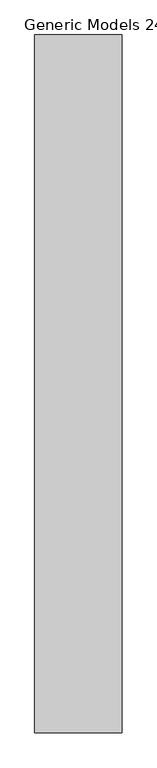
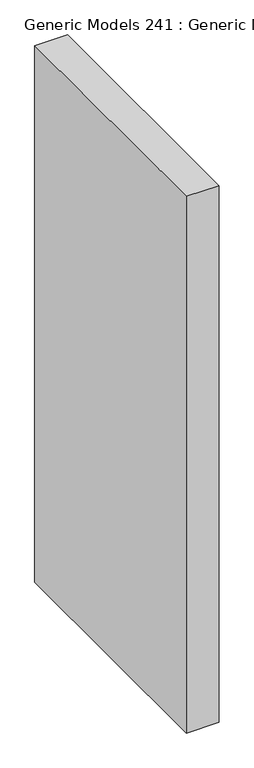
"""IFC4 building model written with IfcOpenShell, lengths in millimetres: proxy geometry, Generic Models 241 : Generic Models 1."""

import ifcopenshell
import ifcopenshell.guid

model = None  # the IFC model being written
_history = None  # IfcOwnerHistory: only IFC2X3 demands one
_inside = {}  # id of a spatial element -> (the spatial element, [elements in it])
_under = {}  # id of a project, library or spatial element -> (it, [spatial elements below it])
_declared = {}  # id of a project -> (the project, [libraries it declares])
_typed = {}  # id of a type object -> (the type object, [elements of that type])
_made_of = {}  # id of a material, layer set ... -> (it, [elements and type objects made of it])


def new_model(schema):
    """Start an empty IFC model of exactly this schema.

    Asked for "IFC4X3", IfcOpenShell would pick the latest addendum, in which some entities
    have other attributes; the version numbers below select the first issue.
    IFC2X3 requires an IfcOwnerHistory on every rooted entity: one is made here for all.
    """
    global model, _history
    if schema == "IFC4X3":
        model = ifcopenshell.file(schema_version=(4, 3, 0, 0))
    else:
        model = ifcopenshell.file(schema=schema)
    _inside.clear()
    _under.clear()
    _declared.clear()
    _typed.clear()
    _made_of.clear()
    _history = None
    if model.schema == "IFC2X3":
        org = make("IfcOrganization", Name="unknown")
        user = make(
            "IfcPersonAndOrganization",
            ThePerson=make("IfcPerson", FamilyName="unknown"),
            TheOrganization=org,
        )
        app = make(
            "IfcApplication",
            ApplicationDeveloper=org,
            Version="unknown",
            ApplicationFullName="unknown",
            ApplicationIdentifier="unknown",
        )
        _history = make(
            "IfcOwnerHistory",
            OwningUser=user,
            OwningApplication=app,
            ChangeAction="ADDED",
            CreationDate=0,
        )
    return model


def make(cls, **values):
    """One entity of the class cls with the attributes given. An attribute that is None is left unset."""
    return model.create_entity(
        cls, **{name: value for name, value in values.items() if value is not None}
    )


def rooted(cls, **values):
    """An entity with a GlobalId (a new one), such as an element, a storey or a relation."""
    return make(cls, GlobalId=ifcopenshell.guid.new(), OwnerHistory=_history, **values)


def si_unit(unit_type, name, prefix=None):
    """IfcSIUnit, for example si_unit("LENGTHUNIT", "METRE", prefix="MILLI")."""
    return make("IfcSIUnit", UnitType=unit_type, Prefix=prefix, Name=name)


def assignment(units):
    """IfcUnitAssignment: the units of a project."""
    return None if units is None else make("IfcUnitAssignment", Units=units)


def point(xyz):
    """IfcCartesianPoint."""
    return None if xyz is None else make("IfcCartesianPoint", Coordinates=xyz)


def direction(xyz):
    """IfcDirection."""
    return None if xyz is None else make("IfcDirection", DirectionRatios=xyz)


def frame(location, z_axis=None, x_axis=None):
    """IfcAxis2Placement3D, a coordinate frame: its origin and axes. An axis left out is left unset."""
    return make(
        "IfcAxis2Placement3D",
        Location=point(location),
        Axis=direction(z_axis),
        RefDirection=direction(x_axis),
    )


def origin():
    """The frame at (0, 0, 0) with its axes left unset."""
    return frame((0.0, 0.0, 0.0))


def place(relative_to, where):
    """IfcLocalPlacement: puts the frame where relative to a parent placement (None: the world)."""
    return make(
        "IfcLocalPlacement", PlacementRelTo=relative_to, RelativePlacement=where
    )


def context(
    kind, dimensions, precision=None, world=None, true_north=None, identifier=None
):
    """IfcGeometricRepresentationContext, for example the 3D "Model" context."""
    return make(
        "IfcGeometricRepresentationContext",
        ContextIdentifier=identifier,
        ContextType=kind,
        CoordinateSpaceDimension=dimensions,
        Precision=precision,
        WorldCoordinateSystem=world,
        TrueNorth=true_north,
    )


def project(units=None, contexts=None):
    """IfcProject with its units and contexts."""
    return rooted(
        "IfcProject",
        Name="project",
        RepresentationContexts=contexts,
        UnitsInContext=assignment(units),
    )


def spatial(cls, under=None, at=None, **own):
    """A site, building, storey or space (cls), placed at a placement, below another one or the project."""
    s = rooted(cls, ObjectPlacement=at, **own)
    if under is not None:
        _under.setdefault(under.id(), (under, []))[1].append(s)
    return s


def polyline(points):
    """IfcPolyline through the points."""
    return make("IfcPolyline", Points=[point(p) for p in points])


def outline(outer, holes=None, kind="AREA"):
    """IfcArbitraryClosedProfileDef: a profile drawn as a closed curve; with holes, ...WithVoids."""
    if holes is None:
        return make("IfcArbitraryClosedProfileDef", ProfileType=kind, OuterCurve=outer)
    return make(
        "IfcArbitraryProfileDefWithVoids",
        ProfileType=kind,
        OuterCurve=outer,
        InnerCurves=holes,
    )


def extrude(swept, where, along, depth):
    """IfcExtrudedAreaSolid: the profile swept, set in the frame where, extruded along a direction by depth."""
    return make(
        "IfcExtrudedAreaSolid",
        SweptArea=swept,
        Position=where,
        ExtrudedDirection=direction(along),
        Depth=depth,
    )


def shape(context_of_items, identifier, shape_type, items):
    """IfcShapeRepresentation: the items that make up one representation, for example the "Body"."""
    return make(
        "IfcShapeRepresentation",
        ContextOfItems=context_of_items,
        RepresentationIdentifier=identifier,
        RepresentationType=shape_type,
        Items=items,
    )


def source(mapping_origin, context_of_items, identifier, shape_type, items):
    """IfcRepresentationMap: a shape defined once, which mapped items show again and again."""
    return make(
        "IfcRepresentationMap",
        MappingOrigin=mapping_origin,
        MappedRepresentation=shape(context_of_items, identifier, shape_type, items),
    )


def transform(
    local_origin,
    x_axis=None,
    y_axis=None,
    z_axis=None,
    scale=None,
    scale2=None,
    scale3=None,
    uniform=True,
):
    """IfcCartesianTransformationOperator3D, or its non-uniform kind. x_axis, y_axis, z_axis: its Axis1, 2, 3."""
    if uniform:
        return make(
            "IfcCartesianTransformationOperator3D",
            Axis1=direction(x_axis),
            Axis2=direction(y_axis),
            LocalOrigin=point(local_origin),
            Scale=scale,
            Axis3=direction(z_axis),
        )
    return make(
        "IfcCartesianTransformationOperator3DnonUniform",
        Axis1=direction(x_axis),
        Axis2=direction(y_axis),
        LocalOrigin=point(local_origin),
        Scale=scale,
        Axis3=direction(z_axis),
        Scale2=scale2,
        Scale3=scale3,
    )


def mapped(mapping_source, mapping_target):
    """IfcMappedItem: shows the shape of a source again, moved by a transform."""
    return make(
        "IfcMappedItem", MappingSource=mapping_source, MappingTarget=mapping_target
    )


def made_of(thing, what):
    """Note that an element or type object is made of a material, layer set ...; save() writes the relation."""
    if what is not None:
        _made_of.setdefault(what.id(), (what, []))[1].append(thing)
    return thing


def element(
    cls,
    number,
    at=None,
    inside=None,
    cuts=None,
    type_object=None,
    material=None,
    context=None,
    identifier="Body",
    shape_type=None,
    held_by="IfcProductDefinitionShape",
    body=None,
    shapes=None,
    **own,
):
    """One element of the class cls, such as IfcWall. Its Tag is "e" and its number.

    at: its placement. inside: the storey or other place that contains it. cuts: it is an
    opening in that element (IfcRelVoidsElement). A single representation is given by context,
    identifier, shape_type and body (its items); several are given by shapes. held_by: the class
    of the entity that holds the representations. save() writes the other relations.
    """
    e = rooted(cls, Tag="e%d" % number, ObjectPlacement=at, **own)
    if body is not None:
        shapes = [shape(context, identifier, shape_type, body)]
    if shapes is not None:
        e.Representation = make(held_by, Representations=shapes)
    if inside is not None:
        _inside.setdefault(inside.id(), (inside, []))[1].append(e)
    if cuts is not None:
        rooted(
            "IfcRelVoidsElement", RelatingBuildingElement=cuts, RelatedOpeningElement=e
        )
    if type_object is not None:
        _typed.setdefault(type_object.id(), (type_object, []))[1].append(e)
    return made_of(e, material)


def aggregate(whole, parts):
    """IfcRelAggregates: a whole, such as a stair, and the parts it consists of."""
    return rooted("IfcRelAggregates", RelatingObject=whole, RelatedObjects=parts)


def save(model, path):
    """Write the relations noted so far, then the file.

    IfcRelAggregates (storeys below a building ...), IfcRelContainedInSpatialStructure (elements
    in a storey), IfcRelDefinesByType, IfcRelAssociatesMaterial and IfcRelDeclares: one each for
    every whole, place, type object, material and project.
    """
    for whole, parts in _under.values():
        aggregate(whole, parts)
    for where, things in _inside.values():
        rooted(
            "IfcRelContainedInSpatialStructure",
            RelatedElements=things,
            RelatingStructure=where,
        )
    for kind, things in _typed.values():
        rooted("IfcRelDefinesByType", RelatedObjects=things, RelatingType=kind)
    for what, things in _made_of.values():
        rooted("IfcRelAssociatesMaterial", RelatedObjects=things, RelatingMaterial=what)
    for by, libraries in _declared.values():
        rooted("IfcRelDeclares", RelatingContext=by, RelatedDefinitions=libraries)
    model.write(path)


def generic_models_241_generic_models_1_d4f8735c(model_context):
    return source(origin(), model_context, "Body", "SweptSolid", [
        extrude(outline(polyline([(48469.55, 1219.2), (48469.55, 0.0), (48317.15, 0.0), (48317.15, 1219.2), (48469.55, 1219.2)])), frame((0.0, 0.0, 3048.0), z_axis=(0.0, 0.0, 1.0), x_axis=(1.0, 0.0, 0.0)), (0.0, 0.0, 1.0), 2633.9569015),
    ])


if __name__ == "__main__":
    model = new_model("IFC4")
    model_context = context("Model", 3, world=origin())
    ifc_project = project(units=[si_unit("LENGTHUNIT", "METRE", prefix="MILLI")], contexts=[model_context])
    site = spatial("IfcSite", under=ifc_project)
    building = spatial("IfcBuilding", under=site)
    placement = place(None, origin())
    generic_models_241_generic_models_1_shape = generic_models_241_generic_models_1_d4f8735c(model_context)
    element("IfcBuildingElementProxy", 1, Name="Generic Models 241 : Generic Models 1", ObjectType="Generic Models 241 : Generic Models 1", at=placement, inside=building, context=model_context, shape_type="MappedRepresentation", body=[
        mapped(generic_models_241_generic_models_1_shape, transform((0.0, 0.0, 0.0), x_axis=(1.0, 0.0, 0.0), y_axis=(0.0, 1.0, 0.0), z_axis=(0.0, 0.0, 1.0))),
    ])
    save(model, "model.ifc")

# Revit data of these elements
# Element 1 (IfcBuildingElementProxy, "Generic Models 241 : Generic Models 1")
#   Materials on its faces: "EXISTING WALL"
# Materials
#   "EXISTING WALL": class "Generic", colour RGB 201 201 201, transparency 0, Cost = 0
